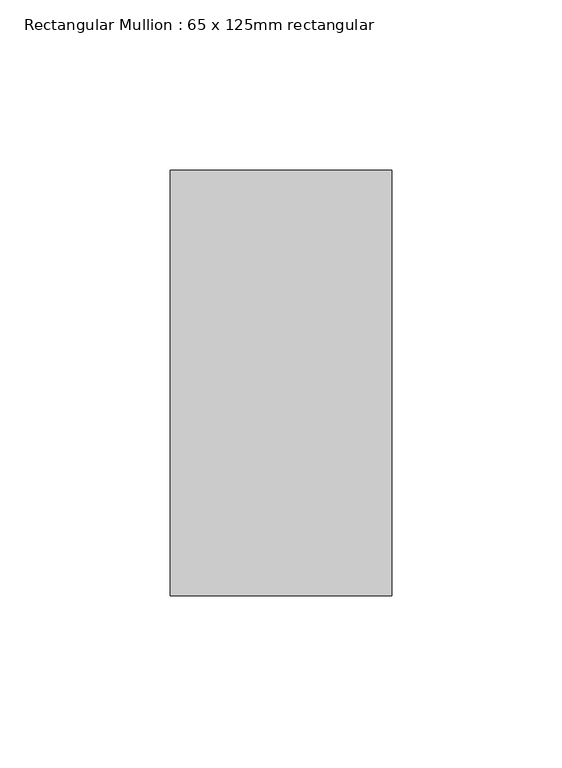
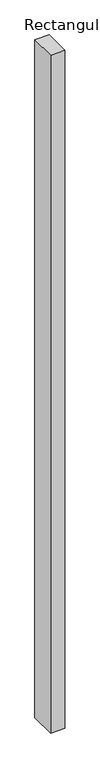
"""IFC4 building model written with IfcOpenShell, lengths in millimetres: member geometry, Rectangular Mullion : 65 x 125mm rectangular."""

from ifc_helpers import new_model, si_unit, frame, origin, place, context, project, spatial, polyline, outline, extrude, source, transform, mapped, element, save


def rectangular_mullion_65_x_125mm_rectangular_bddaf145(model_context):
    return source(origin(), model_context, "Body", "SweptSolid", [
        extrude(outline(polyline([(32.5, 62.5), (32.5, -62.5), (-32.5, -62.5), (-32.5, 62.5), (32.5, 62.5)])), frame((0.0, 0.0, -3300.0), z_axis=(0.0, 0.0, 1.0), x_axis=(1.0, 0.0, 0.0)), (0.0, 0.0, 1.0), 3300.0),
    ])


if __name__ == "__main__":
    model = new_model("IFC4")
    model_context = context("Model", 3, world=origin())
    ifc_project = project(units=[si_unit("LENGTHUNIT", "METRE", prefix="MILLI")], contexts=[model_context])
    site = spatial("IfcSite", under=ifc_project)
    building = spatial("IfcBuilding", under=site)
    placement = place(None, origin())
    rectangular_mullion_65_x_125mm_rectangular_shape = rectangular_mullion_65_x_125mm_rectangular_bddaf145(model_context)
    element("IfcMember", 1, ObjectType="Rectangular Mullion : 65 x 125mm rectangular", at=placement, inside=building, context=model_context, shape_type="MappedRepresentation", body=[
        mapped(rectangular_mullion_65_x_125mm_rectangular_shape, transform((0.0, 0.0, 0.0), x_axis=(1.0, 0.0, 0.0), y_axis=(0.0, 1.0, 0.0), z_axis=(0.0, 0.0, 1.0))),
    ])
    save(model, "model.ifc")

# Revit data of these elements
# Type "Rectangular Mullion : 65 x 125mm rectangular"
#   built-in parameter 1007304 = 0.410105 (stored number, unit not read)
#   built-in parameter 1007301 = 0.106627 (stored number, unit not read)
#   built-in parameter 1007300 = 0.106627 (stored number, unit not read)
# Element 1 (IfcMember, "Rectangular Mullion : 65 x 125mm rectangular")
#   Materials on its faces: "Aluminum"
# Materials
#   "Aluminum": class "Metal", colour RGB 244 245 246, transparency 0, Description = "Aluminum 6061", Cost = 0
